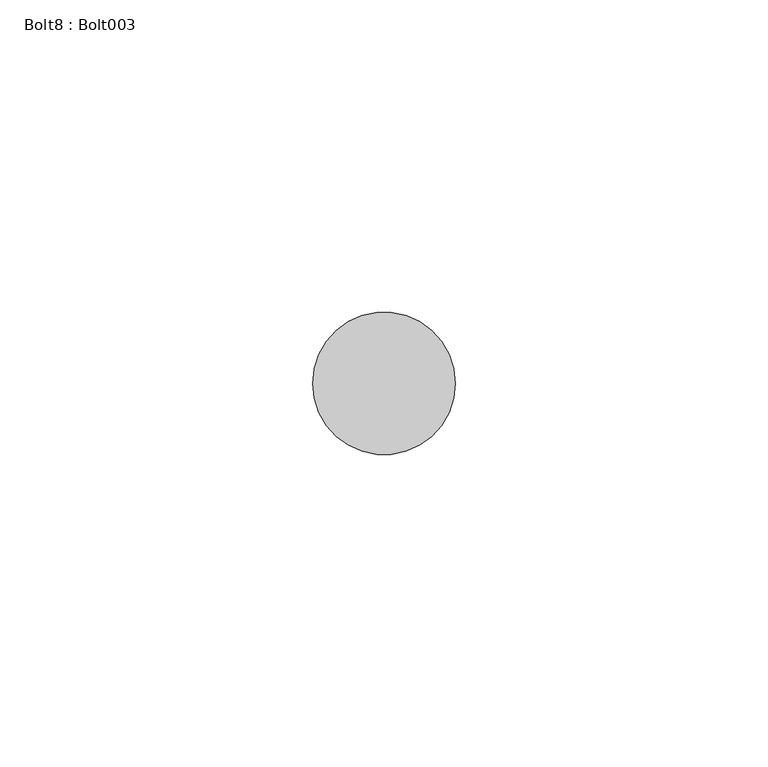
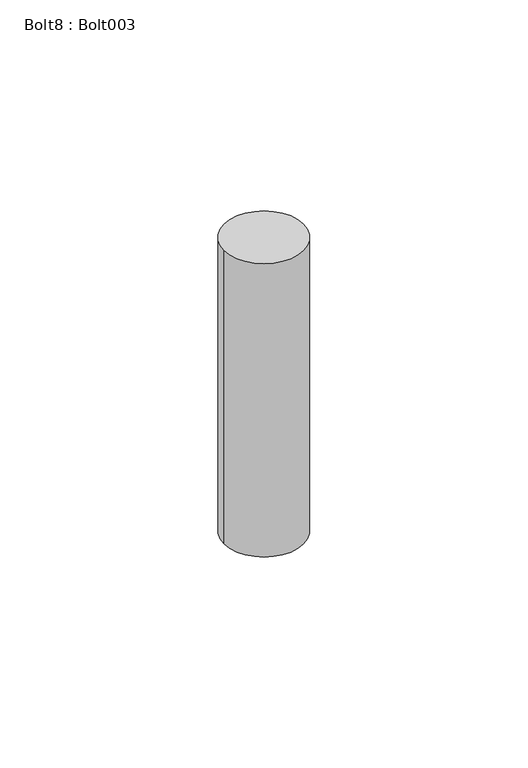
"""IFC4 building model written with IfcOpenShell, lengths in millimetres: proxy geometry, Bolt8 : Bolt003."""

from ifc_helpers import new_model, si_unit, point, frame, frame_2d, origin, place, context, project, spatial, circle_curve, trimmed, segment, composite_curve, outline, extrude, source, transform, mapped, element, save


def bolt8_bolt003_9a242971(model_context):
    return source(origin(), model_context, "Body", "SweptSolid", [
        extrude(outline(composite_curve([segment(trimmed(circle_curve(frame_2d((5027.3346014, 1896.5882072)), 11.4045168), [point((5038.7391183, 1896.5882072))], [point((5015.9300846, 1896.5882072))], False, "CARTESIAN"), True, "CONTINUOUS"), segment(trimmed(circle_curve(frame_2d((5027.3346014, 1896.5882072)), 11.4045168), [point((5015.9300846, 1896.5882072))], [point((5038.7391183, 1896.5882072))], False, "CARTESIAN"), True, "CONTINUOUS")], self_intersect=False)), frame((0.0, 0.0, 36645.5959962), z_axis=(0.0, 0.0, 1.0), x_axis=(1.0, 0.0, 0.0)), (0.0, 0.0, 1.0), 88.9),
    ])


if __name__ == "__main__":
    model = new_model("IFC4")
    model_context = context("Model", 3, world=origin())
    ifc_project = project(units=[si_unit("LENGTHUNIT", "METRE", prefix="MILLI")], contexts=[model_context])
    site = spatial("IfcSite", under=ifc_project)
    building = spatial("IfcBuilding", under=site)
    placement = place(None, origin())
    bolt8_bolt003_shape = bolt8_bolt003_9a242971(model_context)
    element("IfcBuildingElementProxy", 1, Name="Bolt8 : Bolt003", ObjectType="Bolt8 : Bolt003", at=placement, inside=building, context=model_context, shape_type="MappedRepresentation", body=[
        mapped(bolt8_bolt003_shape, transform((0.0, 0.0, 0.0), x_axis=(1.0, 0.0, 0.0), y_axis=(0.0, 1.0, 0.0), z_axis=(0.0, 0.0, 1.0))),
    ])
    save(model, "model.ifc")

# Revit data of these elements
# Type "Bolt8 : Bolt003"
#   NameOverride = "Bolt003"
# Element 1 (IfcBuildingElementProxy, "Bolt8 : Bolt003")
#   Materials on its faces: "TUBE STEEL STRINGER WELDED TO ANCHORED STEEL PLATE - SEE STRUCT DWGS"
# Materials
#   "TUBE STEEL STRINGER WELDED TO ANCHORED STEEL PLATE - SEE STRUCT DWGS": class "Unassigned", colour RGB 128 128 128, transparency 0, Cost = 0
